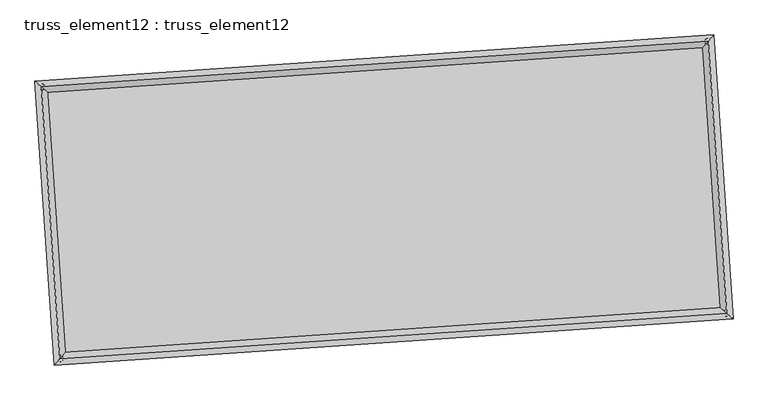
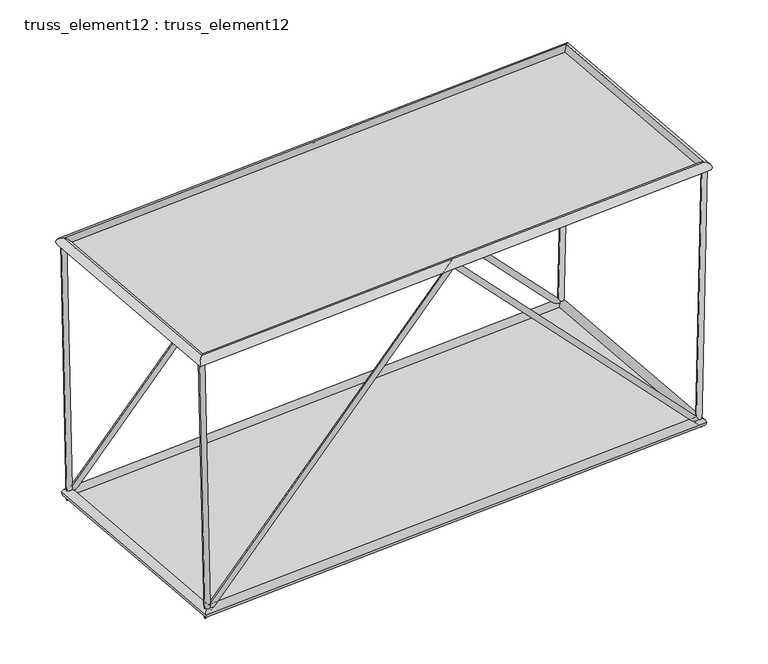
"""IFC4 building model written with IfcOpenShell, lengths in millimetres: plate geometry, truss_element12 : truss_element12."""

from ifc_helpers import new_model, si_unit, frame, origin, origin_with_axes, place, context, project, spatial, polyline, circle_curve, ellipse_curve, outline, extrude, source, transform, mapped, element, save
from ifc_brep_helpers import plane_surface, cylinder_surface, advanced_brep


def truss_element12_truss_element12_301403ea(model_context):
    return source(origin(), model_context, "Body", "SolidModel", [
        advanced_brep(
        [(-3775.2469584, 2268.7026723, 4999.8808289), (-3874.3259881, 2255.3430826, 4997.6746502), (-3667.6082835, 2276.0421444, 121.4057073), (-3761.3785993, 2263.0445357, -121.4057073), (1063.2088881, 2598.6185838, 5070.903767), (1063.6647127, 2592.0458975, 4926.6740735), (5795.0228776, 2921.2629924, 121.4126479), (5889.7380994, 2921.1174961, -121.4126479), (5901.6721346, 2928.5349998, 4999.8930544), (6001.6480134, 2928.7482077, 4997.7071476)],
        [
            (0, 1, circle_curve(frame((-3824.7864732, 2262.0228775, 4998.7777396), z_axis=(-0.022058606365203313, -0.0015040925154301537, 0.9997555479170547), x_axis=(-0.1335964218064517, 0.9910347491932179, -0.0014566990247462872)), 50.0)),
            (1, 0, circle_curve(frame((-3824.7864732, 2262.0228775, 4998.7777396), z_axis=(-0.022058606365203313, -0.0015040925154301537, 0.9997555479170547), x_axis=(-0.1335964218064517, 0.9910347491932179, -0.0014566990247462872)), 50.0)),
            (0, 2),
            (2, 3, ellipse_curve(frame((-3714.4934414, 2269.54334, 0.0), z_axis=(-0.929831833890302, -0.06340169813126974, 0.3624817034806986), x_axis=(0.3616419769436298, 0.02465899167793033, 0.9319908876387853)), 130.5485583, 50.0)),
            (3, 1),
            (3, 2, ellipse_curve(frame((-3714.4934414, 2269.54334, 0.0), z_axis=(-0.929831833890302, -0.06340169813126974, 0.3624817034806986), x_axis=(0.3616419769436298, 0.02465899167793033, 0.9319908876387853)), 130.5485583, 50.0)),
            (2, 4),
            (4, 5, ellipse_curve(frame((1063.4368004, 2595.3322406, 4998.7889203), z_axis=(-0.9976833946750359, -0.06802823813325101, -5.297341116227876e-05), x_axis=(5.2850692750050104e-05, 3.603687834190323e-06, -0.9999999985969089)), 72.2718761, 50.0)),
            (5, 3),
            (5, 4, ellipse_curve(frame((1063.4368004, 2595.3322406, 4998.7889203), z_axis=(-0.9976833946750359, -0.06802823813325101, -5.297341116227876e-05), x_axis=(5.2850692750050104e-05, 3.603687834190323e-06, -0.9999999985969089)), 72.2718761, 50.0)),
            (4, 6),
            (6, 7, ellipse_curve(frame((5842.3804885, 2921.1902443, 0.0), z_axis=(-0.9297759208968333, -0.0633978856367901, -0.3626257644145411), x_axis=(-0.36178570414534755, -0.024668791889457083, 0.931934844816294)), 130.5638727, 50.0)),
            (7, 5),
            (7, 6, ellipse_curve(frame((5842.3804885, 2921.1902443, 0.0), z_axis=(-0.9297759208968333, -0.0633978856367901, -0.3626257644145411), x_axis=(-0.36178570414534755, -0.024668791889457083, 0.931934844816294)), 130.5638727, 50.0)),
            (8, 9, circle_curve(frame((5951.660074, 2928.6416038, 4998.800101), z_axis=(0.021855917096442128, 0.0014902719046874222, 0.9997600201936081), x_axis=(-0.0021641430734946694, 0.9999966166591524, -0.001443313897180082)), 50.0)),
            (9, 8, circle_curve(frame((5951.660074, 2928.6416038, 4998.800101), z_axis=(0.021855917096442128, 0.0014902719046874222, 0.9997600201936081), x_axis=(-0.0021641430734946694, 0.9999966166591524, -0.001443313897180082)), 50.0)),
            (6, 8),
            (9, 7),
        ],
        [
            plane_surface(frame((-3824.7864732, 2312.0228209, 4998.8529625), z_axis=(-0.022058606365203737, -0.0015040925154315642, 0.9997555479170548), x_axis=(0.9997566793401409, -3.318625963721899e-05, 0.022058581401513063))),
            cylinder_surface(frame((-3824.7864732, 2262.0228775, 4998.7777396), z_axis=(-0.022058606365203317, -0.0015040925154301541, 0.9997555479170549), x_axis=(-0.1335964218064517, 0.9910347491932179, -0.0014566990247462872)), 50.0),
            cylinder_surface(frame((-3714.4934414, 2269.54334, 0.0), z_axis=(-0.690191184581497, -0.04706151321429389, -0.7220951064091011), x_axis=(-0.020415630046097626, 0.998752117142888, -0.04557861946592952)), 50.0),
            cylinder_surface(frame((1063.4368004, 2595.3322406, 4998.7889203), z_axis=(-0.6902675071609956, -0.04706671736086042, 0.7220218090020676), x_axis=(-0.11534041081619323, 0.9922795571850488, -0.04558365963144496)), 50.0),
            plane_surface(frame((5951.660074, 2878.6416593, 4998.8746324), z_axis=(0.021855917096441312, 0.0014902719046848058, 0.9997600201936081), x_axis=(0.9997611309147169, -3.257904132603074e-05, -0.02185589281481271))),
            cylinder_surface(frame((5842.3804885, 2921.1902443, 0.0), z_axis=(-0.021855917096442128, -0.0014902719046874222, -0.9997600201936081), x_axis=(-0.0021641430734946694, 0.9999966166591524, -0.001443313897180082)), 50.0),
        ],
        [
            (0, [[1, 2]]),
            (1, [[-1, 3, 4, 5]]),
            (1, [[-2, -5, 6, -3]]),
            (2, [[-4, 7, 8, 9]]),
            (2, [[-6, -9, 10, -7]]),
            (3, [[-8, 11, 12, 13]]),
            (3, [[-10, -13, 14, -11]]),
            (4, [[15, 16]]),
            (5, [[-12, 17, -16, 18]]),
            (5, [[-14, -18, -15, -17]]),
        ],
    ),
        advanced_brep(
        [(-3503.1340054, -1722.030912, 4999.8808289), (-3602.2130352, -1735.3905017, 4997.6746502), (-3395.4953306, -1714.6914399, 121.4057073), (-3489.2656464, -1727.6890486, -121.4057073), (1335.321841, -1392.1150005, 5070.903767), (1335.7776656, -1398.6876868, 4926.6740735), (6067.1358305, -1069.4705919, 121.4126479), (6161.8510524, -1069.6160882, -121.4126479), (6173.7850875, -1062.1985845, 4999.8930544), (6273.7609663, -1061.9853766, 4997.7071476)],
        [
            (0, 1, circle_curve(frame((-3552.6735203, -1728.7107068, 4998.7777396), z_axis=(-0.0220586063652034, -0.0015040925154302146, 0.9997555479170548), x_axis=(-0.13359642180645137, 0.9910347491932178, -0.001456699024746231)), 50.0)),
            (1, 0, circle_curve(frame((-3552.6735203, -1728.7107068, 4998.7777396), z_axis=(-0.0220586063652034, -0.0015040925154302146, 0.9997555479170548), x_axis=(-0.13359642180645137, 0.9910347491932178, -0.001456699024746231)), 50.0)),
            (0, 2),
            (2, 3, ellipse_curve(frame((-3442.3804885, -1721.1902443, 0.0), z_axis=(-0.929831833890302, -0.06340169813126961, 0.3624817034806985), x_axis=(0.3616419769436297, 0.024658991677930217, 0.9319908876387852)), 130.5485583, 50.0)),
            (3, 1),
            (3, 2, ellipse_curve(frame((-3442.3804885, -1721.1902443, 0.0), z_axis=(-0.929831833890302, -0.06340169813126961, 0.3624817034806985), x_axis=(0.3616419769436297, 0.024658991677930217, 0.9319908876387852)), 130.5485583, 50.0)),
            (2, 4),
            (4, 5, ellipse_curve(frame((1335.5497533, -1395.4013437, 4998.7889203), z_axis=(-0.9976833946750359, -0.06802823813325097, -5.297341116235902e-05), x_axis=(5.285069275020386e-05, 3.6036878343633e-06, -0.9999999985969089)), 72.2718761, 50.0)),
            (5, 3),
            (5, 4, ellipse_curve(frame((1335.5497533, -1395.4013437, 4998.7889203), z_axis=(-0.9976833946750359, -0.06802823813325097, -5.297341116235902e-05), x_axis=(5.285069275020386e-05, 3.6036878343633e-06, -0.9999999985969089)), 72.2718761, 50.0)),
            (4, 6),
            (6, 7, ellipse_curve(frame((6114.4934414, -1069.54334, 0.0), z_axis=(-0.9297759208968333, -0.06339788563679019, -0.3626257644145409), x_axis=(-0.36178570414534744, -0.024668791889457125, 0.9319348448162941)), 130.5638727, 50.0)),
            (7, 5),
            (7, 6, ellipse_curve(frame((6114.4934414, -1069.54334, 0.0), z_axis=(-0.9297759208968333, -0.06339788563679019, -0.3626257644145409), x_axis=(-0.36178570414534744, -0.024668791889457125, 0.9319348448162941)), 130.5638727, 50.0)),
            (8, 9, circle_curve(frame((6223.7730269, -1062.0919805, 4998.800101), z_axis=(0.021855917096442214, 0.0014902719046874218, 0.9997600201936081), x_axis=(-0.002164143073494981, 0.9999966166591524, -0.0014433138971800747)), 50.0)),
            (9, 8, circle_curve(frame((6223.7730269, -1062.0919805, 4998.800101), z_axis=(0.021855917096442214, 0.0014902719046874218, 0.9997600201936081), x_axis=(-0.002164143073494981, 0.9999966166591524, -0.0014433138971800747)), 50.0)),
            (6, 8),
            (9, 7),
        ],
        [
            plane_surface(frame((-3552.6735203, -1678.7107634, 4998.8529625), z_axis=(-0.022058606365203737, -0.0015040925154315764, 0.9997555479170548), x_axis=(0.9997566793401409, -3.318625963721899e-05, 0.022058581401513063))),
            cylinder_surface(frame((-3552.6735203, -1728.7107068, 4998.7777396), z_axis=(-0.022058606365203397, -0.0015040925154302142, 0.9997555479170546), x_axis=(-0.13359642180645137, 0.9910347491932178, -0.001456699024746231)), 50.0),
            cylinder_surface(frame((-3442.3804885, -1721.1902443, 0.0), z_axis=(-0.6901911845814968, -0.04706151321429372, -0.7220951064091014), x_axis=(-0.02041563004609754, 0.998752117142888, -0.04557861946592936)), 50.0),
            cylinder_surface(frame((1335.5497533, -1395.4013437, 4998.7889203), z_axis=(-0.6902675071609955, -0.04706671736086049, 0.7220218090020676), x_axis=(-0.11534041081619317, 0.9922795571850488, -0.04558365963144479)), 50.0),
            plane_surface(frame((6223.7730269, -1112.091925, 4998.8746324), z_axis=(0.02185591709644131, 0.001490271904684816, 0.9997600201936081), x_axis=(0.9997611309147169, -3.257904132558665e-05, -0.02185589281481271))),
            cylinder_surface(frame((6114.4934414, -1069.54334, 0.0), z_axis=(-0.021855917096442214, -0.0014902719046874218, -0.9997600201936081), x_axis=(-0.002164143073494981, 0.9999966166591524, -0.0014433138971800747)), 50.0),
        ],
        [
            (0, [[1, 2]]),
            (1, [[-1, 3, 4, 5]]),
            (1, [[-2, -5, 6, -3]]),
            (2, [[-4, 7, 8, 9]]),
            (2, [[-6, -9, 10, -7]]),
            (3, [[-8, 11, 12, 13]]),
            (3, [[-10, -13, 14, -11]]),
            (4, [[15, 16]]),
            (5, [[-12, 17, -16, 18]]),
            (5, [[-14, -18, -15, -17]]),
        ],
    ),
        advanced_brep(
        [(-3552.6677087, -1728.7042655, 4908.7777398), (-3552.679332, -1728.7171481, 5088.7777394), (-3824.7931055, 2262.0284703, 5088.7777394), (-3824.779841, 2262.0172847, 4908.7777398), (5951.6654758, 2928.6480171, 5088.8001008), (5951.6546721, 2928.6351904, 4908.8001012), (6223.7792493, -1062.0976013, 5088.8001008), (6223.7668045, -1062.0863598, 4908.8001012)],
        [
            (0, 1, ellipse_curve(frame((-3552.6735203, -1728.7107068, 4998.7777396), z_axis=(-0.7535719234036206, 0.6573654662782067, -1.6135980941074279e-06), x_axis=(-0.6573654662762446, -0.7535719234053321, -1.6135980941074448e-06)), 127.2792206, 90.0)),
            (1, 2),
            (2, 3, ellipse_curve(frame((-3824.7864732, 2262.0228775, 4998.7777396), z_axis=(-0.6573654662762446, -0.7535719234053322, -1.6135980941074584e-06), x_axis=(0.7535719234036207, -0.6573654662782067, 1.6135980941074419e-06)), 127.2792206, 90.0)),
            (3, 0),
            (1, 0, ellipse_curve(frame((-3552.6735203, -1728.7107068, 4998.7777396), z_axis=(-0.7535719234036206, 0.6573654662782067, -1.6135980941074279e-06), x_axis=(-0.6573654662762446, -0.7535719234053321, -1.6135980941074448e-06)), 127.2792206, 90.0)),
            (3, 2, ellipse_curve(frame((-3824.7864732, 2262.0228775, 4998.7777396), z_axis=(-0.6573654662762446, -0.7535719234053322, -1.6135980941074584e-06), x_axis=(0.7535719234036207, -0.6573654662782067, 1.6135980941074419e-06)), 127.2792206, 90.0)),
            (2, 4),
            (4, 5, ellipse_curve(frame((5951.660074, 2928.6416038, 4998.800101), z_axis=(-0.7535719234036206, 0.6573654662782067, -1.6135980941074558e-06), x_axis=(-0.6573654662762446, -0.753571923405332, -1.6135980941074438e-06)), 127.2792206, 90.0)),
            (5, 3),
            (5, 4, ellipse_curve(frame((5951.660074, 2928.6416038, 4998.800101), z_axis=(-0.7535719234036206, 0.6573654662782067, -1.6135980941074558e-06), x_axis=(-0.6573654662762446, -0.753571923405332, -1.6135980941074438e-06)), 127.2792206, 90.0)),
            (4, 6),
            (6, 7, ellipse_curve(frame((6223.7730269, -1062.0919805, 4998.800101), z_axis=(0.6573654662762446, 0.7535719234053322, 1.6135980941074302e-06), x_axis=(-0.7535719234036207, 0.6573654662782067, -1.6135980941074425e-06)), 127.2792206, 90.0)),
            (7, 5),
            (7, 6, ellipse_curve(frame((6223.7730269, -1062.0919805, 4998.800101), z_axis=(0.6573654662762446, 0.7535719234053322, 1.6135980941074302e-06), x_axis=(-0.7535719234036207, 0.6573654662782067, -1.6135980941074425e-06)), 127.2792206, 90.0)),
            (6, 1),
            (0, 7),
        ],
        [
            cylinder_surface(frame((-3552.6735203, -1728.7107068, 4998.7777396), z_axis=(0.06802823822870047, -0.9976833960748768, 0.0), x_axis=(-0.9976833936796621, -0.06802823806537987, -6.929323564644417e-05)), 90.0),
            cylinder_surface(frame((-3824.7864732, 2262.0228775, 4998.7777396), z_axis=(-0.9976833960722788, -0.06802823822852337, -2.2819723089061332e-06), x_axis=(-0.06802823792339617, 0.997683393845226, -6.701126334266164e-05)), 90.0),
            cylinder_surface(frame((5951.660074, 2928.6416038, 4998.800101), z_axis=(-0.0680282382287004, 0.9976833960748768, 0.0), x_axis=(0.9976833939847893, 0.06802823808618527, -6.472929103887912e-05)), 90.0),
            cylinder_surface(frame((6223.7730269, -1062.0919805, 4998.800101), z_axis=(0.997683396072279, 0.06802823822852329, 2.281972308906114e-06), x_axis=(0.06802823822852329, -0.9976833938244205, -6.701126334266163e-05)), 90.0),
        ],
        [
            (0, [[1, 2, 3, 4]]),
            (0, [[5, -4, 6, -2]]),
            (1, [[-3, 7, 8, 9]]),
            (1, [[-6, -9, 10, -7]]),
            (2, [[-8, 11, 12, 13]]),
            (2, [[-10, -13, 14, -11]]),
            (3, [[-12, 15, -1, 16]]),
            (3, [[-14, -16, -5, -15]]),
        ],
    ),
        advanced_brep(
        [(-3358.7115243, -1625.2761972, 0.0), (-3526.0494527, -1817.1042913, 0.0), (-3810.4074885, 2353.2123043, 0.0), (-3618.5793943, 2185.8743758, 0.0), (5926.0494527, 3017.1042913, 0.0), (5758.7115243, 2825.2761972, 0.0), (6210.4074885, -1153.2123043, 0.0), (6018.5793943, -985.8743758, 0.0)],
        [
            (0, 1, ellipse_curve(frame((-3442.3804885, -1721.1902443, 0.0), z_axis=(-0.7535719234054578, 0.6573654662780809, 0.0), x_axis=(-0.6573654662780808, -0.7535719234054579, 0.0)), 127.2792206, 90.0)),
            (1, 2),
            (2, 3, ellipse_curve(frame((-3714.4934414, 2269.54334, 0.0), z_axis=(-0.6573654662780809, -0.753571923405458, 0.0), x_axis=(0.7535719234054579, -0.6573654662780808, 0.0)), 127.2792206, 90.0)),
            (3, 0),
            (1, 0, ellipse_curve(frame((-3442.3804885, -1721.1902443, 0.0), z_axis=(-0.7535719234054578, 0.6573654662780809, 0.0), x_axis=(-0.6573654662780808, -0.7535719234054579, 0.0)), 127.2792206, 90.0)),
            (3, 2, ellipse_curve(frame((-3714.4934414, 2269.54334, 0.0), z_axis=(-0.6573654662780809, -0.753571923405458, 0.0), x_axis=(0.7535719234054579, -0.6573654662780808, 0.0)), 127.2792206, 90.0)),
            (2, 4),
            (4, 5, ellipse_curve(frame((5842.3804885, 2921.1902443, 0.0), z_axis=(-0.7535719234054578, 0.657365466278081, 0.0), x_axis=(-0.6573654662780812, -0.7535719234054576, 0.0)), 127.2792206, 90.0)),
            (5, 3),
            (5, 4, ellipse_curve(frame((5842.3804885, 2921.1902443, 0.0), z_axis=(-0.7535719234054578, 0.657365466278081, 0.0), x_axis=(-0.6573654662780812, -0.7535719234054576, 0.0)), 127.2792206, 90.0)),
            (4, 6),
            (6, 7, ellipse_curve(frame((6114.4934414, -1069.54334, 0.0), z_axis=(0.657365466278081, 0.7535719234054576, 0.0), x_axis=(-0.7535719234054575, 0.6573654662780813, 0.0)), 127.2792206, 90.0)),
            (7, 5),
            (7, 6, ellipse_curve(frame((6114.4934414, -1069.54334, 0.0), z_axis=(0.657365466278081, 0.7535719234054576, 0.0), x_axis=(-0.7535719234054575, 0.6573654662780813, 0.0)), 127.2792206, 90.0)),
            (6, 1),
            (0, 7),
        ],
        [
            cylinder_surface(frame((-3442.3804885, -1721.1902443, 0.0), z_axis=(0.0680282382287013, -0.9976833960748767, 0.0), x_axis=(-0.9976833960748767, -0.0680282382287013, 0.0)), 90.0),
            cylinder_surface(frame((-3714.4934414, 2269.54334, 0.0), z_axis=(-0.9976833960748767, -0.06802823822870113, 0.0), x_axis=(-0.06802823822870113, 0.9976833960748767, 0.0)), 90.0),
            cylinder_surface(frame((5842.3804885, 2921.1902443, 0.0), z_axis=(-0.06802823822870095, 0.9976833960748767, 0.0), x_axis=(0.9976833960748767, 0.06802823822870095, 0.0)), 90.0),
            cylinder_surface(frame((6114.4934414, -1069.54334, 0.0), z_axis=(0.9976833960748767, 0.06802823822870079, 0.0), x_axis=(0.06802823822870079, -0.9976833960748767, 0.0)), 90.0),
        ],
        [
            (0, [[1, 2, 3, 4]]),
            (0, [[5, -4, 6, -2]]),
            (1, [[-3, 7, 8, 9]]),
            (1, [[-6, -9, 10, -7]]),
            (2, [[-8, 11, 12, 13]]),
            (2, [[-10, -13, 14, -11]]),
            (3, [[-12, 15, -1, 16]]),
            (3, [[-14, -16, -5, -15]]),
        ],
    ),
        extrude(outline(polyline([(-3442.3804885, -1721.1902443), (-3714.4934414, 2269.54334), (5842.3804885, 2921.1902443), (6114.4934414, -1069.54334), (-3442.3804885, -1721.1902443)])), origin_with_axes(), (0.0, 0.0, 1.0), 20.0),
        extrude(outline(polyline([(-2000.0, 4899.5736451), (2000.0, 4899.5736451), (2000.0, -4899.5736452), (-2000.0, -4899.5736452), (-2000.0, 4899.5736451)])), frame((1199.4932768, 599.9654485, 4998.7889203), z_axis=(-2.276685882898288e-06, -1.5523855586156375e-07, 0.9999999999973964), x_axis=(-0.06802823822870063, 0.9976833960748767, 0.0)), (0.0, 0.0, 1.0), 20.0),
    ])


if __name__ == "__main__":
    model = new_model("IFC4")
    model_context = context("Model", 3, world=origin())
    ifc_project = project(units=[si_unit("LENGTHUNIT", "METRE", prefix="MILLI")], contexts=[model_context])
    site = spatial("IfcSite", under=ifc_project)
    building = spatial("IfcBuilding", under=site)
    placement = place(None, origin())
    truss_element12_truss_element12_shape = truss_element12_truss_element12_301403ea(model_context)
    element("IfcPlate", 1, ObjectType="truss_element12 : truss_element12", at=placement, inside=building, context=model_context, shape_type="MappedRepresentation", body=[
        mapped(truss_element12_truss_element12_shape, transform((0.0, 0.0, 0.0), x_axis=(1.0, 0.0, 0.0), y_axis=(0.0, 1.0, 0.0), z_axis=(0.0, 0.0, 1.0))),
    ])
    save(model, "model.ifc")

# Revit data of these elements
# Type "truss_element12 : truss_element12"
#   steellbar1 = 90 mm
#   steelbar2 = 50 mm
#   offset1 = 5000 mm
#   M = Default Roof
# Element 1 (IfcPlate, "truss_element12 : truss_element12")
#   Materials on its faces: "Default Roof"
# Materials
#   "Default Roof": class "Miscellaneous", colour RGB 0 127 0, transparency 0, Comments = "Rendering appearance not upgraded Rendering appearance not upgraded ", Cost = 0
